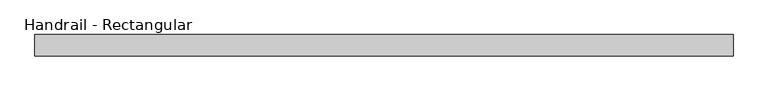
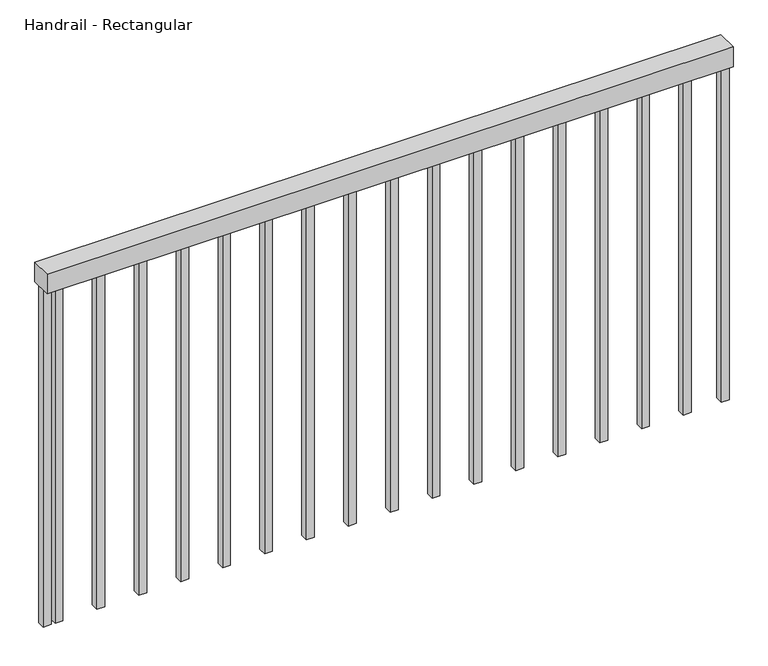
"""IFC4 building model written with IfcOpenShell, lengths in millimetres: railing geometry, Handrail - Rectangular."""

from ifc_helpers import new_model, si_unit, frame, origin, origin_with_axes, place, context, project, spatial, polyline, outline, extrude, source, transform, mapped, element, save


def handrail_rectangular_92c0911c(model_context):
    return source(origin(), model_context, "Body", "SweptSolid", [
        extrude(outline(polyline([(-3832.2086735, -297.4757069), (-3832.2086735, -348.2757069), (-5495.9086735, -348.2757069), (-5495.9086735, -297.4757069), (-3832.2086735, -297.4757069)])), frame((0.0, 0.0, 863.6), z_axis=(0.0, 0.0, 1.0), x_axis=(1.0, 0.0, 0.0)), (0.0, 0.0, 1.0), 50.8),
        extrude(outline(polyline([(-5448.2836735, -313.3507069), (-5448.2836735, -332.4007069), (-5467.3336735, -332.4007069), (-5467.3336735, -313.3507069), (-5448.2836735, -313.3507069)])), origin_with_axes(), (0.0, 0.0, 1.0), 863.6),
        extrude(outline(polyline([(-5346.6836735, -313.3507069), (-5346.6836735, -332.4007069), (-5365.7336735, -332.4007069), (-5365.7336735, -313.3507069), (-5346.6836735, -313.3507069)])), origin_with_axes(), (0.0, 0.0, 1.0), 863.6),
        extrude(outline(polyline([(-5245.0836735, -313.3507069), (-5245.0836735, -332.4007069), (-5264.1336735, -332.4007069), (-5264.1336735, -313.3507069), (-5245.0836735, -313.3507069)])), origin_with_axes(), (0.0, 0.0, 1.0), 863.6),
        extrude(outline(polyline([(-5143.4836735, -313.3507069), (-5143.4836735, -332.4007069), (-5162.5336735, -332.4007069), (-5162.5336735, -313.3507069), (-5143.4836735, -313.3507069)])), origin_with_axes(), (0.0, 0.0, 1.0), 863.6),
        extrude(outline(polyline([(-5041.8836735, -313.3507069), (-5041.8836735, -332.4007069), (-5060.9336735, -332.4007069), (-5060.9336735, -313.3507069), (-5041.8836735, -313.3507069)])), origin_with_axes(), (0.0, 0.0, 1.0), 863.6),
        extrude(outline(polyline([(-4940.2836735, -313.3507069), (-4940.2836735, -332.4007069), (-4959.3336735, -332.4007069), (-4959.3336735, -313.3507069), (-4940.2836735, -313.3507069)])), origin_with_axes(), (0.0, 0.0, 1.0), 863.6),
        extrude(outline(polyline([(-4838.6836735, -313.3507069), (-4838.6836735, -332.4007069), (-4857.7336735, -332.4007069), (-4857.7336735, -313.3507069), (-4838.6836735, -313.3507069)])), origin_with_axes(), (0.0, 0.0, 1.0), 863.6),
        extrude(outline(polyline([(-4737.0836735, -313.3507069), (-4737.0836735, -332.4007069), (-4756.1336735, -332.4007069), (-4756.1336735, -313.3507069), (-4737.0836735, -313.3507069)])), origin_with_axes(), (0.0, 0.0, 1.0), 863.6),
        extrude(outline(polyline([(-4635.4836735, -313.3507069), (-4635.4836735, -332.4007069), (-4654.5336735, -332.4007069), (-4654.5336735, -313.3507069), (-4635.4836735, -313.3507069)])), origin_with_axes(), (0.0, 0.0, 1.0), 863.6),
        extrude(outline(polyline([(-4533.8836735, -313.3507069), (-4533.8836735, -332.4007069), (-4552.9336735, -332.4007069), (-4552.9336735, -313.3507069), (-4533.8836735, -313.3507069)])), origin_with_axes(), (0.0, 0.0, 1.0), 863.6),
        extrude(outline(polyline([(-4432.2836735, -313.3507069), (-4432.2836735, -332.4007069), (-4451.3336735, -332.4007069), (-4451.3336735, -313.3507069), (-4432.2836735, -313.3507069)])), origin_with_axes(), (0.0, 0.0, 1.0), 863.6),
        extrude(outline(polyline([(-4330.6836735, -313.3507069), (-4330.6836735, -332.4007069), (-4349.7336735, -332.4007069), (-4349.7336735, -313.3507069), (-4330.6836735, -313.3507069)])), origin_with_axes(), (0.0, 0.0, 1.0), 863.6),
        extrude(outline(polyline([(-4229.0836735, -313.3507069), (-4229.0836735, -332.4007069), (-4248.1336735, -332.4007069), (-4248.1336735, -313.3507069), (-4229.0836735, -313.3507069)])), origin_with_axes(), (0.0, 0.0, 1.0), 863.6),
        extrude(outline(polyline([(-4127.4836735, -313.3507069), (-4127.4836735, -332.4007069), (-4146.5336735, -332.4007069), (-4146.5336735, -313.3507069), (-4127.4836735, -313.3507069)])), origin_with_axes(), (0.0, 0.0, 1.0), 863.6),
        extrude(outline(polyline([(-4025.8836735, -313.3507069), (-4025.8836735, -332.4007069), (-4044.9336735, -332.4007069), (-4044.9336735, -313.3507069), (-4025.8836735, -313.3507069)])), origin_with_axes(), (0.0, 0.0, 1.0), 863.6),
        extrude(outline(polyline([(-3924.2836735, -313.3507069), (-3924.2836735, -332.4007069), (-3943.3336735, -332.4007069), (-3943.3336735, -313.3507069), (-3924.2836735, -313.3507069)])), origin_with_axes(), (0.0, 0.0, 1.0), 863.6),
        extrude(outline(polyline([(-5476.8586735, -313.3507069), (-5476.8586735, -332.4007069), (-5495.9086735, -332.4007069), (-5495.9086735, -313.3507069), (-5476.8586735, -313.3507069)])), origin_with_axes(), (0.0, 0.0, 1.0), 863.6),
        extrude(outline(polyline([(-3832.2086735, -313.3507069), (-3832.2086735, -332.4007069), (-3851.2586735, -332.4007069), (-3851.2586735, -313.3507069), (-3832.2086735, -313.3507069)])), origin_with_axes(), (0.0, 0.0, 1.0), 863.6),
    ])


if __name__ == "__main__":
    model = new_model("IFC4")
    model_context = context("Model", 3, world=origin())
    ifc_project = project(units=[si_unit("LENGTHUNIT", "METRE", prefix="MILLI")], contexts=[model_context])
    site = spatial("IfcSite", under=ifc_project)
    building = spatial("IfcBuilding", under=site)
    placement = place(None, origin())
    handrail_rectangular_shape = handrail_rectangular_92c0911c(model_context)
    element("IfcRailing", 1, ObjectType="Handrail - Rectangular", at=placement, inside=building, context=model_context, shape_type="MappedRepresentation", body=[
        mapped(handrail_rectangular_shape, transform((0.0, 0.0, 0.0), x_axis=(1.0, 0.0, 0.0), y_axis=(0.0, 1.0, 0.0), z_axis=(0.0, 0.0, 1.0))),
    ])
    save(model, "model.ifc")
